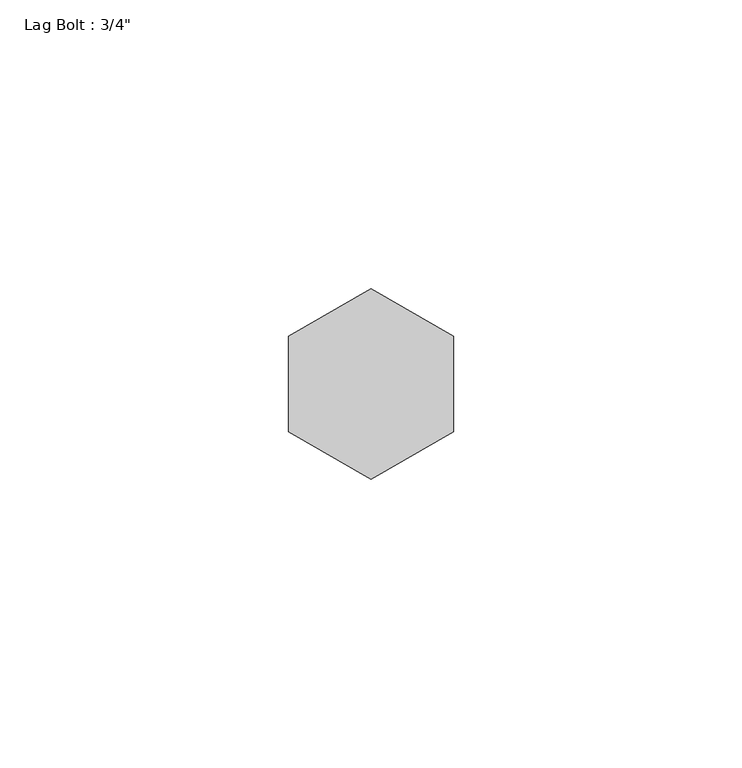
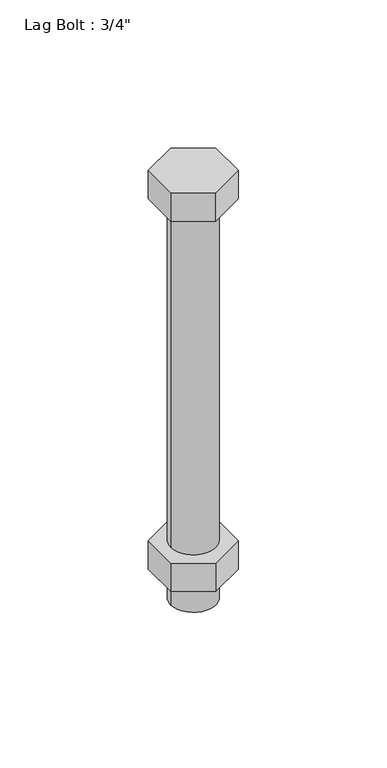
"""IFC4 building model written with IfcOpenShell, lengths in millimetres: proxy geometry."""

import ifcopenshell
import ifcopenshell.guid

model = None  # the IFC model being written
_history = None  # IfcOwnerHistory: only IFC2X3 demands one
_inside = {}  # id of a spatial element -> (the spatial element, [elements in it])
_under = {}  # id of a project, library or spatial element -> (it, [spatial elements below it])
_declared = {}  # id of a project -> (the project, [libraries it declares])
_typed = {}  # id of a type object -> (the type object, [elements of that type])
_made_of = {}  # id of a material, layer set ... -> (it, [elements and type objects made of it])


def new_model(schema):
    """Start an empty IFC model of exactly this schema.

    Asked for "IFC4X3", IfcOpenShell would pick the latest addendum, in which some entities
    have other attributes; the version numbers below select the first issue.
    IFC2X3 requires an IfcOwnerHistory on every rooted entity: one is made here for all.
    """
    global model, _history
    if schema == "IFC4X3":
        model = ifcopenshell.file(schema_version=(4, 3, 0, 0))
    else:
        model = ifcopenshell.file(schema=schema)
    _inside.clear()
    _under.clear()
    _declared.clear()
    _typed.clear()
    _made_of.clear()
    _history = None
    if model.schema == "IFC2X3":
        org = make("IfcOrganization", Name="unknown")
        user = make(
            "IfcPersonAndOrganization",
            ThePerson=make("IfcPerson", FamilyName="unknown"),
            TheOrganization=org,
        )
        app = make(
            "IfcApplication",
            ApplicationDeveloper=org,
            Version="unknown",
            ApplicationFullName="unknown",
            ApplicationIdentifier="unknown",
        )
        _history = make(
            "IfcOwnerHistory",
            OwningUser=user,
            OwningApplication=app,
            ChangeAction="ADDED",
            CreationDate=0,
        )
    return model


def make(cls, **values):
    """One entity of the class cls with the attributes given. An attribute that is None is left unset."""
    return model.create_entity(
        cls, **{name: value for name, value in values.items() if value is not None}
    )


def rooted(cls, **values):
    """An entity with a GlobalId (a new one), such as an element, a storey or a relation."""
    return make(cls, GlobalId=ifcopenshell.guid.new(), OwnerHistory=_history, **values)


def si_unit(unit_type, name, prefix=None):
    """IfcSIUnit, for example si_unit("LENGTHUNIT", "METRE", prefix="MILLI")."""
    return make("IfcSIUnit", UnitType=unit_type, Prefix=prefix, Name=name)


def assignment(units):
    """IfcUnitAssignment: the units of a project."""
    return None if units is None else make("IfcUnitAssignment", Units=units)


def point(xyz):
    """IfcCartesianPoint."""
    return None if xyz is None else make("IfcCartesianPoint", Coordinates=xyz)


def direction(xyz):
    """IfcDirection."""
    return None if xyz is None else make("IfcDirection", DirectionRatios=xyz)


def frame(location, z_axis=None, x_axis=None):
    """IfcAxis2Placement3D, a coordinate frame: its origin and axes. An axis left out is left unset."""
    return make(
        "IfcAxis2Placement3D",
        Location=point(location),
        Axis=direction(z_axis),
        RefDirection=direction(x_axis),
    )


def frame_2d(location, x_axis=None):
    """IfcAxis2Placement2D, a coordinate frame in the plane: its origin and x axis."""
    return make(
        "IfcAxis2Placement2D", Location=point(location), RefDirection=direction(x_axis)
    )


def origin():
    """The frame at (0, 0, 0) with its axes left unset."""
    return frame((0.0, 0.0, 0.0))


def origin_with_axes():
    """The frame at (0, 0, 0) with the z axis (0, 0, 1) and the x axis (1, 0, 0) written out."""
    return frame((0.0, 0.0, 0.0), z_axis=(0.0, 0.0, 1.0), x_axis=(1.0, 0.0, 0.0))


def origin_2d():
    """The frame at (0, 0) in the plane with its x axis left unset."""
    return frame_2d((0.0, 0.0))


def place(relative_to, where):
    """IfcLocalPlacement: puts the frame where relative to a parent placement (None: the world)."""
    return make(
        "IfcLocalPlacement", PlacementRelTo=relative_to, RelativePlacement=where
    )


def context(
    kind, dimensions, precision=None, world=None, true_north=None, identifier=None
):
    """IfcGeometricRepresentationContext, for example the 3D "Model" context."""
    return make(
        "IfcGeometricRepresentationContext",
        ContextIdentifier=identifier,
        ContextType=kind,
        CoordinateSpaceDimension=dimensions,
        Precision=precision,
        WorldCoordinateSystem=world,
        TrueNorth=true_north,
    )


def project(units=None, contexts=None):
    """IfcProject with its units and contexts."""
    return rooted(
        "IfcProject",
        Name="project",
        RepresentationContexts=contexts,
        UnitsInContext=assignment(units),
    )


def spatial(cls, under=None, at=None, **own):
    """A site, building, storey or space (cls), placed at a placement, below another one or the project."""
    s = rooted(cls, ObjectPlacement=at, **own)
    if under is not None:
        _under.setdefault(under.id(), (under, []))[1].append(s)
    return s


def polyline(points):
    """IfcPolyline through the points."""
    return make("IfcPolyline", Points=[point(p) for p in points])


def circle_curve(where, radius):
    """IfcCircle in the frame where."""
    return make("IfcCircle", Position=where, Radius=radius)


def trimmed(basis, trim1, trim2, sense, master):
    """IfcTrimmedCurve: the piece of a basis curve between two trims."""
    return make(
        "IfcTrimmedCurve",
        BasisCurve=basis,
        Trim1=trim1,
        Trim2=trim2,
        SenseAgreement=sense,
        MasterRepresentation=master,
    )


def segment(curve, same_sense, transition):
    """IfcCompositeCurveSegment."""
    return make(
        "IfcCompositeCurveSegment",
        Transition=transition,
        SameSense=same_sense,
        ParentCurve=curve,
    )


def composite_curve(segments, self_intersect=None):
    """IfcCompositeCurve: segments joined end to end."""
    return make("IfcCompositeCurve", Segments=segments, SelfIntersect=self_intersect)


def outline(outer, holes=None, kind="AREA"):
    """IfcArbitraryClosedProfileDef: a profile drawn as a closed curve; with holes, ...WithVoids."""
    if holes is None:
        return make("IfcArbitraryClosedProfileDef", ProfileType=kind, OuterCurve=outer)
    return make(
        "IfcArbitraryProfileDefWithVoids",
        ProfileType=kind,
        OuterCurve=outer,
        InnerCurves=holes,
    )


def extrude(swept, where, along, depth):
    """IfcExtrudedAreaSolid: the profile swept, set in the frame where, extruded along a direction by depth."""
    return make(
        "IfcExtrudedAreaSolid",
        SweptArea=swept,
        Position=where,
        ExtrudedDirection=direction(along),
        Depth=depth,
    )


def shape(context_of_items, identifier, shape_type, items):
    """IfcShapeRepresentation: the items that make up one representation, for example the "Body"."""
    return make(
        "IfcShapeRepresentation",
        ContextOfItems=context_of_items,
        RepresentationIdentifier=identifier,
        RepresentationType=shape_type,
        Items=items,
    )


def source(mapping_origin, context_of_items, identifier, shape_type, items):
    """IfcRepresentationMap: a shape defined once, which mapped items show again and again."""
    return make(
        "IfcRepresentationMap",
        MappingOrigin=mapping_origin,
        MappedRepresentation=shape(context_of_items, identifier, shape_type, items),
    )


def transform(
    local_origin,
    x_axis=None,
    y_axis=None,
    z_axis=None,
    scale=None,
    scale2=None,
    scale3=None,
    uniform=True,
):
    """IfcCartesianTransformationOperator3D, or its non-uniform kind. x_axis, y_axis, z_axis: its Axis1, 2, 3."""
    if uniform:
        return make(
            "IfcCartesianTransformationOperator3D",
            Axis1=direction(x_axis),
            Axis2=direction(y_axis),
            LocalOrigin=point(local_origin),
            Scale=scale,
            Axis3=direction(z_axis),
        )
    return make(
        "IfcCartesianTransformationOperator3DnonUniform",
        Axis1=direction(x_axis),
        Axis2=direction(y_axis),
        LocalOrigin=point(local_origin),
        Scale=scale,
        Axis3=direction(z_axis),
        Scale2=scale2,
        Scale3=scale3,
    )


def mapped(mapping_source, mapping_target):
    """IfcMappedItem: shows the shape of a source again, moved by a transform."""
    return make(
        "IfcMappedItem", MappingSource=mapping_source, MappingTarget=mapping_target
    )


def made_of(thing, what):
    """Note that an element or type object is made of a material, layer set ...; save() writes the relation."""
    if what is not None:
        _made_of.setdefault(what.id(), (what, []))[1].append(thing)
    return thing


def element(
    cls,
    number,
    at=None,
    inside=None,
    cuts=None,
    type_object=None,
    material=None,
    context=None,
    identifier="Body",
    shape_type=None,
    held_by="IfcProductDefinitionShape",
    body=None,
    shapes=None,
    **own,
):
    """One element of the class cls, such as IfcWall. Its Tag is "e" and its number.

    at: its placement. inside: the storey or other place that contains it. cuts: it is an
    opening in that element (IfcRelVoidsElement). A single representation is given by context,
    identifier, shape_type and body (its items); several are given by shapes. held_by: the class
    of the entity that holds the representations. save() writes the other relations.
    """
    e = rooted(cls, Tag="e%d" % number, ObjectPlacement=at, **own)
    if body is not None:
        shapes = [shape(context, identifier, shape_type, body)]
    if shapes is not None:
        e.Representation = make(held_by, Representations=shapes)
    if inside is not None:
        _inside.setdefault(inside.id(), (inside, []))[1].append(e)
    if cuts is not None:
        rooted(
            "IfcRelVoidsElement", RelatingBuildingElement=cuts, RelatedOpeningElement=e
        )
    if type_object is not None:
        _typed.setdefault(type_object.id(), (type_object, []))[1].append(e)
    return made_of(e, material)


def aggregate(whole, parts):
    """IfcRelAggregates: a whole, such as a stair, and the parts it consists of."""
    return rooted("IfcRelAggregates", RelatingObject=whole, RelatedObjects=parts)


def save(model, path):
    """Write the relations noted so far, then the file.

    IfcRelAggregates (storeys below a building ...), IfcRelContainedInSpatialStructure (elements
    in a storey), IfcRelDefinesByType, IfcRelAssociatesMaterial and IfcRelDeclares: one each for
    every whole, place, type object, material and project.
    """
    for whole, parts in _under.values():
        aggregate(whole, parts)
    for where, things in _inside.values():
        rooted(
            "IfcRelContainedInSpatialStructure",
            RelatedElements=things,
            RelatingStructure=where,
        )
    for kind, things in _typed.values():
        rooted("IfcRelDefinesByType", RelatedObjects=things, RelatingType=kind)
    for what, things in _made_of.values():
        rooted("IfcRelAssociatesMaterial", RelatedObjects=things, RelatingMaterial=what)
    for by, libraries in _declared.values():
        rooted("IfcRelDeclares", RelatingContext=by, RelatedDefinitions=libraries)
    model.write(path)


def proxy_709d5af4(model_context):
    return source(origin(), model_context, "Body", "SweptSolid", [
        extrude(outline(polyline([(-14.2875, 8.248892), (0.0, 16.4977839), (14.2875, 8.248892), (14.2875, -8.248892), (0.0, -16.4977839), (-14.2875, -8.248892), (-14.2875, 8.248892)])), frame((0.0, 0.0, -165.1), z_axis=(0.0, 0.0, 1.0), x_axis=(1.0, 0.0, 0.0)), (0.0, 0.0, 1.0), 12.7),
        extrude(outline(polyline([(-14.2875, -8.248892), (-14.2875, 8.248892), (0.0, 16.4977839), (14.2875, 8.248892), (14.2875, -8.248892), (0.0, -16.4977839), (-14.2875, -8.248892)])), origin_with_axes(), (0.0, 0.0, 1.0), 12.7),
        extrude(outline(composite_curve([segment(trimmed(circle_curve(origin_2d(), 9.525), [point((-9.525, 0.0))], [point((9.525, 0.0))], False, "CARTESIAN"), True, "CONTINUOUS"), segment(trimmed(circle_curve(origin_2d(), 9.525), [point((9.525, 0.0))], [point((-9.525, 0.0))], False, "CARTESIAN"), True, "CONTINUOUS")], self_intersect=False)), frame((0.0, 0.0, -177.8), z_axis=(0.0, 0.0, 1.0), x_axis=(1.0, 0.0, 0.0)), (0.0, 0.0, 1.0), 177.8),
    ])


if __name__ == "__main__":
    model = new_model("IFC4")
    model_context = context("Model", 3, world=origin())
    ifc_project = project(units=[si_unit("LENGTHUNIT", "METRE", prefix="MILLI")], contexts=[model_context])
    site = spatial("IfcSite", under=ifc_project)
    building = spatial("IfcBuilding", under=site)
    placement = place(None, origin())
    proxy_shape = proxy_709d5af4(model_context)
    element("IfcBuildingElementProxy", 1, Name="Lag Bolt : 3/4\"", ObjectType="Lag Bolt : 3/4\"", at=placement, inside=building, context=model_context, shape_type="MappedRepresentation", body=[
        mapped(proxy_shape, transform((0.0, 0.0, 0.0), x_axis=(1.0, 0.0, 0.0), y_axis=(0.0, 1.0, 0.0), z_axis=(0.0, 0.0, 1.0))),
    ])
    save(model, "model.ifc")

# Revit data of these elements
# Type "Lag Bolt : 3/4\""
#   Thickness_of_Substrate [instance default] = 0' - 1"
#   Side = 0' - 0.65039"
#   Radius = 0' - 0 3/8"
#   Length = 0' - 7"
#   Head Size = 0' - 1 1/8"
#   Head Radius = 0' - 0 9/16"
#   Head Height = 0' - 0 1/2"
#   Diameter = 0' - 0 3/4"
#   Default Elevation = 4' - 0"
#   Nut_Visibility [instance default] = yes
#   Bolt Material (Size) [instance default] = 5/8" GALV. ANCHOR BOLT @ 24" O.C. (6" MIN. EMBEDMENT)
# Element 1 (IfcBuildingElementProxy, "Lag Bolt : 3/4\"")
#   Thickness_of_Substrate = 0' - 6"
#   Bolt Material (Size) = 3/4" THU BOLT (RAW STEEL)
#   Materials on its faces: "3/4\" THU BOLT (RAW STEEL)"
# Materials
#   "5/8\" GALV. ANCHOR BOLT @ 24\" O.C. (6\" MIN. EMBEDMENT)": class "Generic", colour RGB 120 120 120, transparency 0, Cost = 0
#   "3/4\" THU BOLT (RAW STEEL)": class "Generic", colour RGB 120 120 120, transparency 0, Cost = 0
